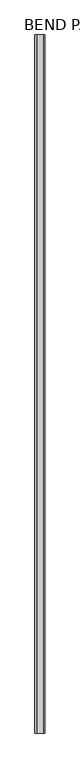
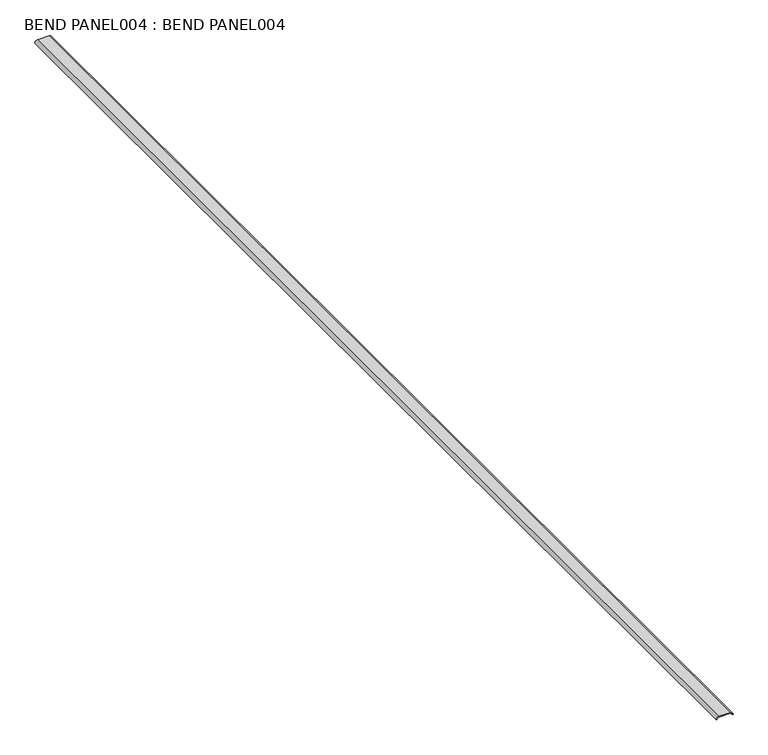
"""IFC4 building model written with IfcOpenShell, lengths in millimetres: proxy geometry, BEND PANEL004 : BEND PANEL004."""

from ifc_helpers import new_model, si_unit, point, frame, frame_2d, origin, place, context, project, spatial, polyline, circle_curve, trimmed, segment, composite_curve, outline, extrude, source, transform, mapped, element, save


def bend_panel004_bend_panel004_15d214a6(model_context):
    return source(origin(), model_context, "Body", "SweptSolid", [
        extrude(outline(composite_curve([segment(polyline([(42576.61192, 5858.4004637), (42576.61192, 5859.5910887)]), True, "CONTINUOUS"), segment(trimmed(circle_curve(frame_2d((42576.6119199, 5862.9993652)), 3.4082764), [point((42576.61192, 5859.5910887))], [point((42580.0201795, 5863.0100787))], True, "CARTESIAN"), True, "CONTINUOUS"), segment(polyline([(42580.0201795, 5863.0100787), (42580.0201963, 5882.3645691)]), True, "CONTINUOUS"), segment(trimmed(circle_curve(frame_2d((42576.6119199, 5882.3645721)), 3.4082764), [point((42580.0201963, 5882.3645691))], [point((42576.61192, 5885.7728485))], True, "CARTESIAN"), True, "CONTINUOUS"), segment(polyline([(42576.61192, 5885.7728485), (42576.61192, 5886.9634735)]), True, "CONTINUOUS"), segment(trimmed(circle_curve(frame_2d((42576.6119199, 5882.3645721)), 4.5989014), [point((42576.61192, 5886.9634735))], [point((42581.2108213, 5882.364568))], False, "CARTESIAN"), True, "CONTINUOUS"), segment(polyline([(42581.2108213, 5882.364568), (42581.2108045, 5863.0118181)]), True, "CONTINUOUS"), segment(trimmed(circle_curve(frame_2d((42576.6119199, 5862.9993652)), 4.5989014), [point((42581.2108045, 5863.0118181))], [point((42576.61192, 5858.4004637))], False, "CARTESIAN"), True, "CONTINUOUS")], self_intersect=False)), frame((0.0, -1052.8906574, 0.0), z_axis=(0.0, 1.0, 0.0), x_axis=(0.0, 0.0, 1.0)), (0.0, 0.0, 1.0), 1999.85),
    ])


if __name__ == "__main__":
    model = new_model("IFC4")
    model_context = context("Model", 3, world=origin())
    ifc_project = project(units=[si_unit("LENGTHUNIT", "METRE", prefix="MILLI")], contexts=[model_context])
    site = spatial("IfcSite", under=ifc_project)
    building = spatial("IfcBuilding", under=site)
    placement = place(None, origin())
    bend_panel004_bend_panel004_shape = bend_panel004_bend_panel004_15d214a6(model_context)
    element("IfcBuildingElementProxy", 1, Name="BEND PANEL004 : BEND PANEL004", ObjectType="BEND PANEL004 : BEND PANEL004", at=placement, inside=building, context=model_context, shape_type="MappedRepresentation", body=[
        mapped(bend_panel004_bend_panel004_shape, transform((0.0, 0.0, 0.0), x_axis=(1.0, 0.0, 0.0), y_axis=(0.0, 1.0, 0.0), z_axis=(0.0, 0.0, 1.0))),
    ])
    save(model, "model.ifc")

# Revit data of these elements
# Type "BEND PANEL004 : BEND PANEL004"
#   NameOverride = "BEND PANEL004"
# Element 1 (IfcBuildingElementProxy, "BEND PANEL004 : BEND PANEL004")
#   Materials on its faces: "METAL PROFILE"
# Materials
#   "METAL PROFILE": class "Unassigned", colour RGB 128 128 128, transparency 0
